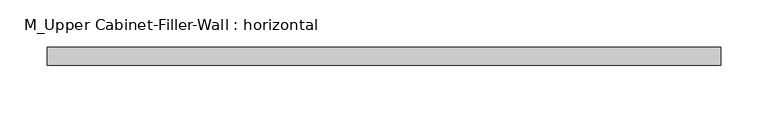
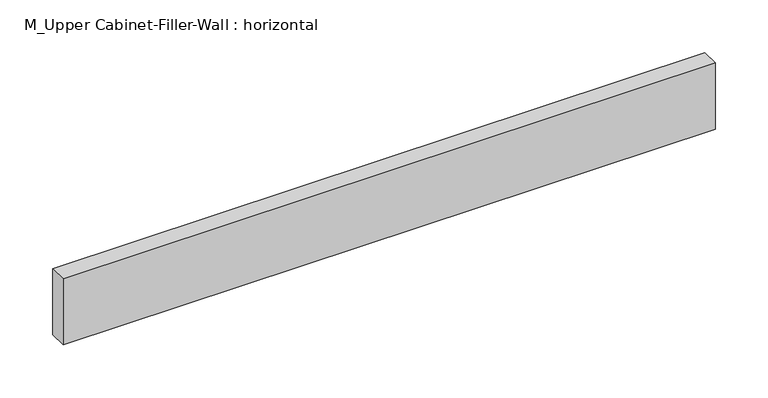
"""IFC4 building model written with IfcOpenShell, lengths in millimetres: furniture geometry, M_Upper Cabinet-Filler-Wall : horizontal."""

from ifc_helpers import new_model, si_unit, frame, origin, place, context, project, spatial, polyline, outline, extrude, source, transform, mapped, element, save


def m_upper_cabinet_filler_wall_horizontal_0d8bff8c(model_context):
    return source(origin(), model_context, "Body", "SweptSolid", [
        extrude(outline(polyline([(-325.8288372, 38.1), (-325.8288372, 57.15), (385.3711628, 57.15), (385.3711628, 38.1), (-325.8288372, 38.1)])), frame((0.0, 0.0, 1923.8), z_axis=(0.0, 0.0, 1.0), x_axis=(1.0, 0.0, 0.0)), (0.0, 0.0, 1.0), 76.2),
    ])


if __name__ == "__main__":
    model = new_model("IFC4")
    model_context = context("Model", 3, world=origin())
    ifc_project = project(units=[si_unit("LENGTHUNIT", "METRE", prefix="MILLI")], contexts=[model_context])
    site = spatial("IfcSite", under=ifc_project)
    building = spatial("IfcBuilding", under=site)
    placement = place(None, origin())
    m_upper_cabinet_filler_wall_horizontal_shape = m_upper_cabinet_filler_wall_horizontal_0d8bff8c(model_context)
    element("IfcFurniture", 1, ObjectType="M_Upper Cabinet-Filler-Wall : horizontal", at=placement, inside=building, context=model_context, shape_type="MappedRepresentation", body=[
        mapped(m_upper_cabinet_filler_wall_horizontal_shape, transform((0.0, 0.0, 0.0), x_axis=(1.0, 0.0, 0.0), y_axis=(0.0, 1.0, 0.0), z_axis=(0.0, 0.0, 1.0))),
    ])
    save(model, "model.ifc")

# Revit data of these elements
# Type "M_Upper Cabinet-Filler-Wall : horizontal"
#   Depth = 0' - 1"
#   Height = 0' - 3"
#   Top Of Cabinet = 6' - 6.74016"
#   Width = 2' - 4"
#   Cabinet Material = none
#   Default Elevation = 0
# Element 1 (IfcFurniture, "M_Upper Cabinet-Filler-Wall : horizontal")
#   Materials on its faces: "Cabinets"
# Materials
#   "Cabinets": class "Miscellaneous", colour RGB 249 249 249, transparency 0
